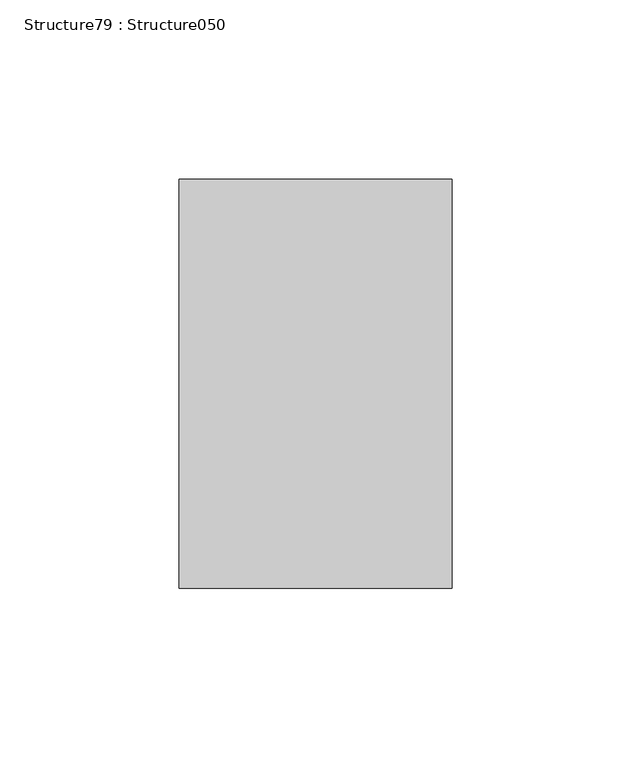
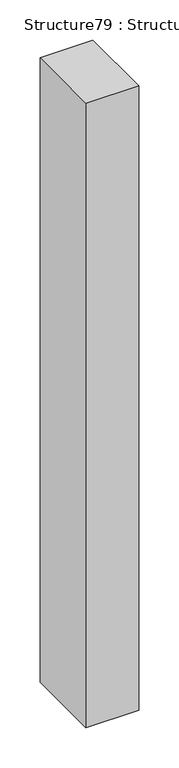
"""IFC4 building model written with IfcOpenShell, lengths in millimetres: proxy geometry, Structure79 : Structure050."""

from ifc_helpers import new_model, si_unit, frame, origin, place, context, project, spatial, polyline, outline, extrude, source, transform, mapped, element, save


def structure79_structure050_91c7bec2(model_context):
    return source(origin(), model_context, "Body", "SweptSolid", [
        extrude(outline(polyline([(-59031.6926606, 282570.0454107), (-59031.6926606, 282684.2815472), (-58955.4926606, 282684.2815472), (-58955.4926606, 282570.0454107), (-59031.6926606, 282570.0454107)])), frame((0.0, 0.0, 3528.5825142), z_axis=(0.0, 0.0, 1.0), x_axis=(1.0, 0.0, 0.0)), (0.0, 0.0, 1.0), 951.8594804),
    ])


if __name__ == "__main__":
    model = new_model("IFC4")
    model_context = context("Model", 3, world=origin())
    ifc_project = project(units=[si_unit("LENGTHUNIT", "METRE", prefix="MILLI")], contexts=[model_context])
    site = spatial("IfcSite", under=ifc_project)
    building = spatial("IfcBuilding", under=site)
    placement = place(None, origin())
    structure79_structure050_shape = structure79_structure050_91c7bec2(model_context)
    element("IfcBuildingElementProxy", 1, Name="Structure79 : Structure050", ObjectType="Structure79 : Structure050", at=placement, inside=building, context=model_context, shape_type="MappedRepresentation", body=[
        mapped(structure79_structure050_shape, transform((0.0, 0.0, 0.0), x_axis=(1.0, 0.0, 0.0), y_axis=(0.0, 1.0, 0.0), z_axis=(0.0, 0.0, 1.0))),
    ])
    save(model, "model.ifc")

# Revit data of these elements
# Type "Structure79 : Structure050"
#   NameOverride = "Structure050"
# Element 1 (IfcBuildingElementProxy, "Structure79 : Structure050")
#   Materials on its faces: "BRUSHED ALUM. LETTERING"
# Materials
#   "BRUSHED ALUM. LETTERING": class "Unassigned", colour RGB 169 181 186, transparency 0, Cost = 0
